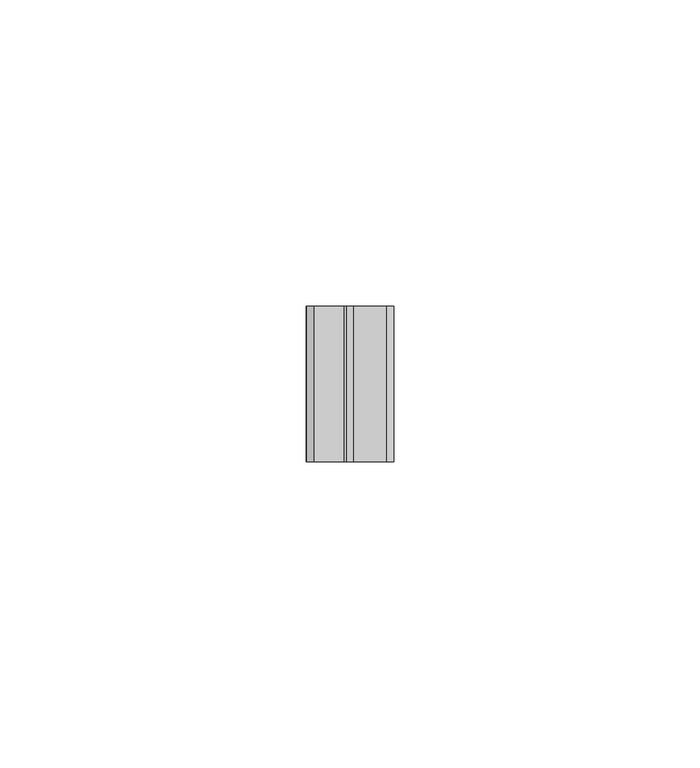
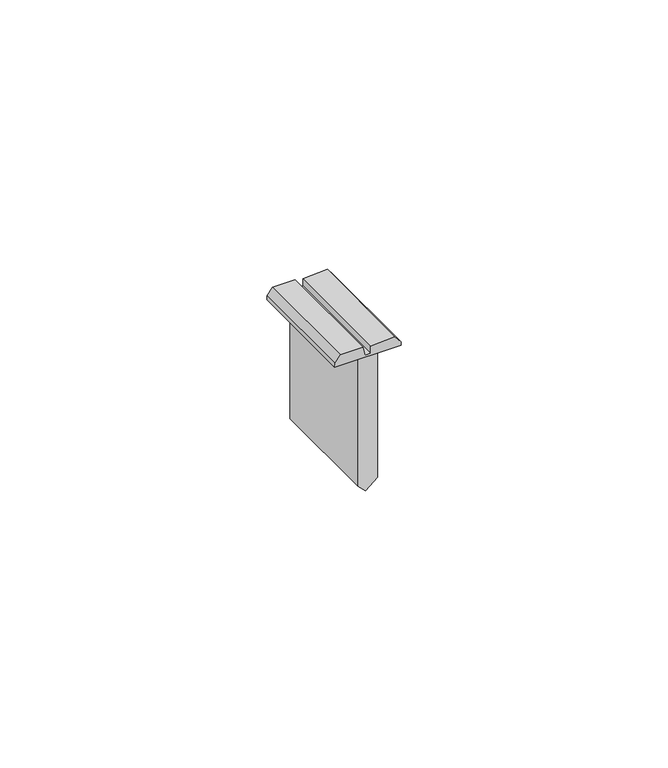
"""IFC4 building model written with IfcOpenShell, lengths in millimetres: proxy geometry, FASTENER2:FASTENER006:297428 : FASTENER2:FASTENER006:297428."""

from ifc_helpers import new_model, si_unit, frame, origin, place, context, project, spatial, polyline, outline, extrude, source, transform, mapped, element, save


def generic_models_613513fb(model_context):
    return source(origin(), model_context, "Body", "SweptSolid", [
        extrude(outline(polyline([(42577.1576024, 10642.6545919), (42577.1576024, 10656.9508971), (42577.9674245, 10656.9508971), (42579.5612959, 10655.712195), (42579.1650604, 10650.4265129), (42577.5756297, 10650.4265129), (42577.5756297, 10649.179408), (42579.587761, 10648.7831725), (42579.587761, 10643.9040906), (42577.9938896, 10642.6653885), (42577.1576024, 10642.6545919)])), frame((0.0, -799.9581163, 0.0), z_axis=(0.0, 1.0, 0.0), x_axis=(0.0, 0.0, 1.0)), (0.0, 0.0, 1.0), 25.4),
        extrude(outline(polyline([(42577.1576024, 10651.90503), (42577.1576024, 10647.6981115), (42548.1988623, 10647.6981115), (42546.5833096, 10649.355126), (42548.7638676, 10651.90503), (42577.1576024, 10651.90503)])), frame((0.0, -799.9581163, 0.0), z_axis=(0.0, 1.0, 0.0), x_axis=(0.0, 0.0, 1.0)), (0.0, 0.0, 1.0), 25.4),
    ])


if __name__ == "__main__":
    model = new_model("IFC4")
    model_context = context("Model", 3, world=origin())
    ifc_project = project(units=[si_unit("LENGTHUNIT", "METRE", prefix="MILLI")], contexts=[model_context])
    site = spatial("IfcSite", under=ifc_project)
    building = spatial("IfcBuilding", under=site)
    placement = place(None, origin())
    generic_models_shape = generic_models_613513fb(model_context)
    element("IfcBuildingElementProxy", 1, Name="FASTENER2:FASTENER006:297428 : FASTENER2:FASTENER006:297428", ObjectType="FASTENER2:FASTENER006:297428 : FASTENER2:FASTENER006:297428", at=placement, inside=building, context=model_context, shape_type="MappedRepresentation", body=[
        mapped(generic_models_shape, transform((0.0, 0.0, 0.0), x_axis=(1.0, 0.0, 0.0), y_axis=(0.0, 1.0, 0.0), z_axis=(0.0, 0.0, 1.0))),
    ])
    save(model, "model.ifc")

# Revit data of these elements
# Type "FASTENER2:FASTENER006:297428 : FASTENER2:FASTENER006:297428"
#   NameOverride = "FASTENER2:FASTENER006:297428"
#   ObjectTypeOverride = "FASTENER2:FASTENER006"
#   Reference = "FASTENER006"
#   Category = "Generic Models"
#   Tag = "297428"
# Element 1 (IfcBuildingElementProxy, "FASTENER2:FASTENER006:297428 : FASTENER2:FASTENER006:297428")
#   Materials on its faces: "ENGINEERED PANCAKE HEAD FASTENER @ 12\" O.C."
# Materials
#   "ENGINEERED PANCAKE HEAD FASTENER @ 12\" O.C.": class "Unassigned", colour RGB 255 255 255, transparency 0, Cost = 0
